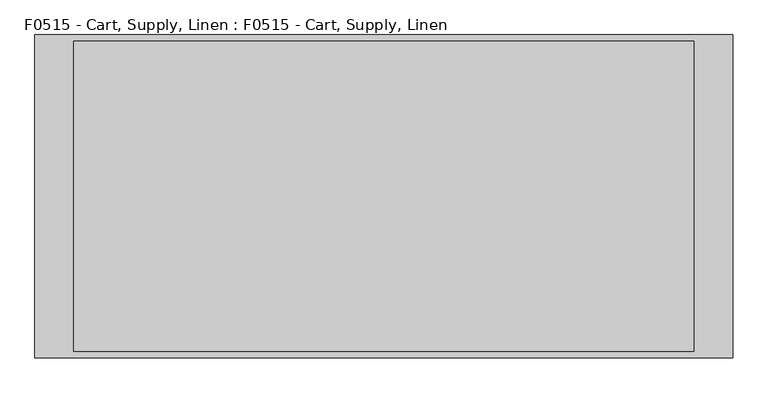
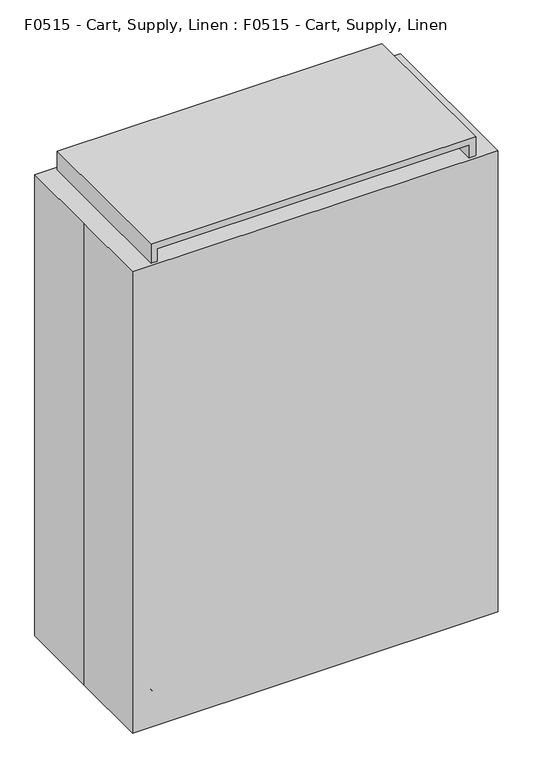
"""IFC4 building model written with IfcOpenShell, lengths in millimetres: proxy geometry, F0515 - Cart, Supply, Linen : F0515 - Cart, Supply, Linen."""

import ifcopenshell
import ifcopenshell.guid

model = None  # the IFC model being written
_history = None  # IfcOwnerHistory: only IFC2X3 demands one
_inside = {}  # id of a spatial element -> (the spatial element, [elements in it])
_under = {}  # id of a project, library or spatial element -> (it, [spatial elements below it])
_declared = {}  # id of a project -> (the project, [libraries it declares])
_typed = {}  # id of a type object -> (the type object, [elements of that type])
_made_of = {}  # id of a material, layer set ... -> (it, [elements and type objects made of it])


def new_model(schema):
    """Start an empty IFC model of exactly this schema.

    Asked for "IFC4X3", IfcOpenShell would pick the latest addendum, in which some entities
    have other attributes; the version numbers below select the first issue.
    IFC2X3 requires an IfcOwnerHistory on every rooted entity: one is made here for all.
    """
    global model, _history
    if schema == "IFC4X3":
        model = ifcopenshell.file(schema_version=(4, 3, 0, 0))
    else:
        model = ifcopenshell.file(schema=schema)
    _inside.clear()
    _under.clear()
    _declared.clear()
    _typed.clear()
    _made_of.clear()
    _history = None
    if model.schema == "IFC2X3":
        org = make("IfcOrganization", Name="unknown")
        user = make(
            "IfcPersonAndOrganization",
            ThePerson=make("IfcPerson", FamilyName="unknown"),
            TheOrganization=org,
        )
        app = make(
            "IfcApplication",
            ApplicationDeveloper=org,
            Version="unknown",
            ApplicationFullName="unknown",
            ApplicationIdentifier="unknown",
        )
        _history = make(
            "IfcOwnerHistory",
            OwningUser=user,
            OwningApplication=app,
            ChangeAction="ADDED",
            CreationDate=0,
        )
    return model


def make(cls, **values):
    """One entity of the class cls with the attributes given. An attribute that is None is left unset."""
    return model.create_entity(
        cls, **{name: value for name, value in values.items() if value is not None}
    )


def rooted(cls, **values):
    """An entity with a GlobalId (a new one), such as an element, a storey or a relation."""
    return make(cls, GlobalId=ifcopenshell.guid.new(), OwnerHistory=_history, **values)


def si_unit(unit_type, name, prefix=None):
    """IfcSIUnit, for example si_unit("LENGTHUNIT", "METRE", prefix="MILLI")."""
    return make("IfcSIUnit", UnitType=unit_type, Prefix=prefix, Name=name)


def assignment(units):
    """IfcUnitAssignment: the units of a project."""
    return None if units is None else make("IfcUnitAssignment", Units=units)


def point(xyz):
    """IfcCartesianPoint."""
    return None if xyz is None else make("IfcCartesianPoint", Coordinates=xyz)


def direction(xyz):
    """IfcDirection."""
    return None if xyz is None else make("IfcDirection", DirectionRatios=xyz)


def frame(location, z_axis=None, x_axis=None):
    """IfcAxis2Placement3D, a coordinate frame: its origin and axes. An axis left out is left unset."""
    return make(
        "IfcAxis2Placement3D",
        Location=point(location),
        Axis=direction(z_axis),
        RefDirection=direction(x_axis),
    )


def frame_2d(location, x_axis=None):
    """IfcAxis2Placement2D, a coordinate frame in the plane: its origin and x axis."""
    return make(
        "IfcAxis2Placement2D", Location=point(location), RefDirection=direction(x_axis)
    )


def origin():
    """The frame at (0, 0, 0) with its axes left unset."""
    return frame((0.0, 0.0, 0.0))


def origin_with_axes():
    """The frame at (0, 0, 0) with the z axis (0, 0, 1) and the x axis (1, 0, 0) written out."""
    return frame((0.0, 0.0, 0.0), z_axis=(0.0, 0.0, 1.0), x_axis=(1.0, 0.0, 0.0))


def place(relative_to, where):
    """IfcLocalPlacement: puts the frame where relative to a parent placement (None: the world)."""
    return make(
        "IfcLocalPlacement", PlacementRelTo=relative_to, RelativePlacement=where
    )


def context(
    kind, dimensions, precision=None, world=None, true_north=None, identifier=None
):
    """IfcGeometricRepresentationContext, for example the 3D "Model" context."""
    return make(
        "IfcGeometricRepresentationContext",
        ContextIdentifier=identifier,
        ContextType=kind,
        CoordinateSpaceDimension=dimensions,
        Precision=precision,
        WorldCoordinateSystem=world,
        TrueNorth=true_north,
    )


def project(units=None, contexts=None):
    """IfcProject with its units and contexts."""
    return rooted(
        "IfcProject",
        Name="project",
        RepresentationContexts=contexts,
        UnitsInContext=assignment(units),
    )


def spatial(cls, under=None, at=None, **own):
    """A site, building, storey or space (cls), placed at a placement, below another one or the project."""
    s = rooted(cls, ObjectPlacement=at, **own)
    if under is not None:
        _under.setdefault(under.id(), (under, []))[1].append(s)
    return s


def polyline(points):
    """IfcPolyline through the points."""
    return make("IfcPolyline", Points=[point(p) for p in points])


def circle_curve(where, radius):
    """IfcCircle in the frame where."""
    return make("IfcCircle", Position=where, Radius=radius)


def trimmed(basis, trim1, trim2, sense, master):
    """IfcTrimmedCurve: the piece of a basis curve between two trims."""
    return make(
        "IfcTrimmedCurve",
        BasisCurve=basis,
        Trim1=trim1,
        Trim2=trim2,
        SenseAgreement=sense,
        MasterRepresentation=master,
    )


def segment(curve, same_sense, transition):
    """IfcCompositeCurveSegment."""
    return make(
        "IfcCompositeCurveSegment",
        Transition=transition,
        SameSense=same_sense,
        ParentCurve=curve,
    )


def composite_curve(segments, self_intersect=None):
    """IfcCompositeCurve: segments joined end to end."""
    return make("IfcCompositeCurve", Segments=segments, SelfIntersect=self_intersect)


def outline(outer, holes=None, kind="AREA"):
    """IfcArbitraryClosedProfileDef: a profile drawn as a closed curve; with holes, ...WithVoids."""
    if holes is None:
        return make("IfcArbitraryClosedProfileDef", ProfileType=kind, OuterCurve=outer)
    return make(
        "IfcArbitraryProfileDefWithVoids",
        ProfileType=kind,
        OuterCurve=outer,
        InnerCurves=holes,
    )


def extrude(swept, where, along, depth):
    """IfcExtrudedAreaSolid: the profile swept, set in the frame where, extruded along a direction by depth."""
    return make(
        "IfcExtrudedAreaSolid",
        SweptArea=swept,
        Position=where,
        ExtrudedDirection=direction(along),
        Depth=depth,
    )


def faces_of(points, faces, orient=None, outer=None):
    """IfcFace entities. A face is a list of loops; a loop is a list of indices into points, from 0.

    orient and outer hold one flag for each loop. By default every Orientation is true, the
    first loop of a face is its IfcFaceOuterBound and the others are IfcFaceBound.
    """
    made = []
    for i, loops in enumerate(faces):
        bounds = []
        for j, loop in enumerate(loops):
            is_outer = j == 0 if outer is None else outer[i][j]
            bounds.append(
                make(
                    "IfcFaceOuterBound" if is_outer else "IfcFaceBound",
                    Bound=make("IfcPolyLoop", Polygon=[points[k] for k in loop]),
                    Orientation=True if orient is None else orient[i][j],
                )
            )
        made.append(make("IfcFace", Bounds=bounds))
    return made


def faceted_brep(points, faces, orient=None, outer=None, voids=None):
    """IfcFacetedBrep: a solid bounded by flat faces; with voids (closed shells), ...WithVoids."""
    shared = [point(p) for p in points]
    hull = make("IfcClosedShell", CfsFaces=faces_of(shared, faces, orient, outer))
    if voids is None:
        return make("IfcFacetedBrep", Outer=hull)
    return make(
        "IfcFacetedBrepWithVoids",
        Outer=hull,
        Voids=[
            make(cls, CfsFaces=faces_of(shared, fs, o, b)) for cls, fs, o, b in voids
        ],
    )


def shape(context_of_items, identifier, shape_type, items):
    """IfcShapeRepresentation: the items that make up one representation, for example the "Body"."""
    return make(
        "IfcShapeRepresentation",
        ContextOfItems=context_of_items,
        RepresentationIdentifier=identifier,
        RepresentationType=shape_type,
        Items=items,
    )


def source(mapping_origin, context_of_items, identifier, shape_type, items):
    """IfcRepresentationMap: a shape defined once, which mapped items show again and again."""
    return make(
        "IfcRepresentationMap",
        MappingOrigin=mapping_origin,
        MappedRepresentation=shape(context_of_items, identifier, shape_type, items),
    )


def transform(
    local_origin,
    x_axis=None,
    y_axis=None,
    z_axis=None,
    scale=None,
    scale2=None,
    scale3=None,
    uniform=True,
):
    """IfcCartesianTransformationOperator3D, or its non-uniform kind. x_axis, y_axis, z_axis: its Axis1, 2, 3."""
    if uniform:
        return make(
            "IfcCartesianTransformationOperator3D",
            Axis1=direction(x_axis),
            Axis2=direction(y_axis),
            LocalOrigin=point(local_origin),
            Scale=scale,
            Axis3=direction(z_axis),
        )
    return make(
        "IfcCartesianTransformationOperator3DnonUniform",
        Axis1=direction(x_axis),
        Axis2=direction(y_axis),
        LocalOrigin=point(local_origin),
        Scale=scale,
        Axis3=direction(z_axis),
        Scale2=scale2,
        Scale3=scale3,
    )


def mapped(mapping_source, mapping_target):
    """IfcMappedItem: shows the shape of a source again, moved by a transform."""
    return make(
        "IfcMappedItem", MappingSource=mapping_source, MappingTarget=mapping_target
    )


def made_of(thing, what):
    """Note that an element or type object is made of a material, layer set ...; save() writes the relation."""
    if what is not None:
        _made_of.setdefault(what.id(), (what, []))[1].append(thing)
    return thing


def element(
    cls,
    number,
    at=None,
    inside=None,
    cuts=None,
    type_object=None,
    material=None,
    context=None,
    identifier="Body",
    shape_type=None,
    held_by="IfcProductDefinitionShape",
    body=None,
    shapes=None,
    **own,
):
    """One element of the class cls, such as IfcWall. Its Tag is "e" and its number.

    at: its placement. inside: the storey or other place that contains it. cuts: it is an
    opening in that element (IfcRelVoidsElement). A single representation is given by context,
    identifier, shape_type and body (its items); several are given by shapes. held_by: the class
    of the entity that holds the representations. save() writes the other relations.
    """
    e = rooted(cls, Tag="e%d" % number, ObjectPlacement=at, **own)
    if body is not None:
        shapes = [shape(context, identifier, shape_type, body)]
    if shapes is not None:
        e.Representation = make(held_by, Representations=shapes)
    if inside is not None:
        _inside.setdefault(inside.id(), (inside, []))[1].append(e)
    if cuts is not None:
        rooted(
            "IfcRelVoidsElement", RelatingBuildingElement=cuts, RelatedOpeningElement=e
        )
    if type_object is not None:
        _typed.setdefault(type_object.id(), (type_object, []))[1].append(e)
    return made_of(e, material)


def aggregate(whole, parts):
    """IfcRelAggregates: a whole, such as a stair, and the parts it consists of."""
    return rooted("IfcRelAggregates", RelatingObject=whole, RelatedObjects=parts)


def save(model, path):
    """Write the relations noted so far, then the file.

    IfcRelAggregates (storeys below a building ...), IfcRelContainedInSpatialStructure (elements
    in a storey), IfcRelDefinesByType, IfcRelAssociatesMaterial and IfcRelDeclares: one each for
    every whole, place, type object, material and project.
    """
    for whole, parts in _under.values():
        aggregate(whole, parts)
    for where, things in _inside.values():
        rooted(
            "IfcRelContainedInSpatialStructure",
            RelatedElements=things,
            RelatingStructure=where,
        )
    for kind, things in _typed.values():
        rooted("IfcRelDefinesByType", RelatedObjects=things, RelatingType=kind)
    for what, things in _made_of.values():
        rooted("IfcRelAssociatesMaterial", RelatedObjects=things, RelatingMaterial=what)
    for by, libraries in _declared.values():
        rooted("IfcRelDeclares", RelatingContext=by, RelatedDefinitions=libraries)
    model.write(path)


def f0515_cart_supply_linen_f0515_cart_supply_linen_772906bd(model_context):
    return source(origin(), model_context, "Body", "SolidModel", [
        extrude(outline(polyline([(138.1125, 609.6), (138.1125, 496.8875), (60.3746094, 542.8753906), (60.3746094, 555.5753906), (138.1125, 609.6)])), frame((0.0, 241.3, 0.0), z_axis=(0.0, 1.0, 0.0), x_axis=(0.0, 0.0, 1.0)), (0.0, 0.0, 1.0), 3.175),
        extrude(outline(polyline([(138.1125, 609.6), (138.1125, 496.8875), (60.3746094, 542.8753906), (60.3746094, 555.5753906), (138.1125, 609.6)])), frame((0.0, 263.525, 0.0), z_axis=(0.0, 1.0, 0.0), x_axis=(0.0, 0.0, 1.0)), (0.0, 0.0, 1.0), 3.175),
        extrude(outline(composite_curve([segment(trimmed(circle_curve(frame_2d((60.3746094, 549.2253906)), 60.3746094), [point((60.3746094, 609.6))], [point((60.3746094, 488.8507812))], False, "CARTESIAN"), True, "CONTINUOUS"), segment(trimmed(circle_curve(frame_2d((60.3746094, 549.2253906)), 60.3746094), [point((60.3746094, 488.8507812))], [point((60.3746094, 609.6))], False, "CARTESIAN"), True, "CONTINUOUS")], self_intersect=False)), frame((0.0, 244.475, 0.0), z_axis=(0.0, 1.0, 0.0), x_axis=(0.0, 0.0, 1.0)), (0.0, 0.0, 1.0), 19.05),
        extrude(outline(composite_curve([segment(trimmed(circle_curve(frame_2d((584.2, 279.4)), 25.4), [point((584.2, 304.8))], [point((609.6, 279.4))], False, "CARTESIAN"), True, "CONTINUOUS"), segment(polyline([(609.6, 279.4), (609.6, 228.6)]), True, "CONTINUOUS"), segment(trimmed(circle_curve(frame_2d((584.2, 228.6)), 25.4), [point((609.6, 228.6))], [point((584.2, 203.2))], False, "CARTESIAN"), True, "CONTINUOUS"), segment(polyline([(584.2, 203.2), (533.4, 203.2)]), True, "CONTINUOUS"), segment(trimmed(circle_curve(frame_2d((533.4, 228.6)), 25.4), [point((533.4, 203.2))], [point((508.0, 228.6))], False, "CARTESIAN"), True, "CONTINUOUS"), segment(polyline([(508.0, 228.6), (508.0, 279.4)]), True, "CONTINUOUS"), segment(trimmed(circle_curve(frame_2d((533.4, 279.4)), 25.4), [point((508.0, 279.4))], [point((533.4, 304.8))], False, "CARTESIAN"), True, "CONTINUOUS"), segment(polyline([(533.4, 304.8), (584.2, 304.8)]), True, "CONTINUOUS")], self_intersect=False)), frame((0.0, 0.0, 138.1125), z_axis=(0.0, 0.0, 1.0), x_axis=(1.0, 0.0, 0.0)), (0.0, 0.0, 1.0), 25.4),
        extrude(outline(polyline([(138.1125, -609.6), (60.3746094, -555.5753906), (60.3746094, -542.8753906), (138.1125, -496.8875), (138.1125, -609.6)])), frame((0.0, 241.3, 0.0), z_axis=(0.0, 1.0, 0.0), x_axis=(0.0, 0.0, 1.0)), (0.0, 0.0, 1.0), 3.175),
        extrude(outline(polyline([(138.1125, -609.6), (60.3746094, -555.5753906), (60.3746094, -542.8753906), (138.1125, -496.8875), (138.1125, -609.6)])), frame((0.0, 263.525, 0.0), z_axis=(0.0, 1.0, 0.0), x_axis=(0.0, 0.0, 1.0)), (0.0, 0.0, 1.0), 3.175),
        extrude(outline(composite_curve([segment(trimmed(circle_curve(frame_2d((60.3746094, -549.2253906)), 60.3746094), [point((60.3746094, -609.6))], [point((60.3746094, -488.8507812))], False, "CARTESIAN"), True, "CONTINUOUS"), segment(trimmed(circle_curve(frame_2d((60.3746094, -549.2253906)), 60.3746094), [point((60.3746094, -488.8507812))], [point((60.3746094, -609.6))], False, "CARTESIAN"), True, "CONTINUOUS")], self_intersect=False)), frame((0.0, 244.475, 0.0), z_axis=(0.0, 1.0, 0.0), x_axis=(0.0, 0.0, 1.0)), (0.0, 0.0, 1.0), 19.05),
        extrude(outline(composite_curve([segment(polyline([(-584.2, 304.8), (-533.4, 304.8)]), True, "CONTINUOUS"), segment(trimmed(circle_curve(frame_2d((-533.4, 279.4)), 25.4), [point((-533.4, 304.8))], [point((-508.0, 279.4))], False, "CARTESIAN"), True, "CONTINUOUS"), segment(polyline([(-508.0, 279.4), (-508.0, 228.6)]), True, "CONTINUOUS"), segment(trimmed(circle_curve(frame_2d((-533.4, 228.6)), 25.4), [point((-508.0, 228.6))], [point((-533.4, 203.2))], False, "CARTESIAN"), True, "CONTINUOUS"), segment(polyline([(-533.4, 203.2), (-584.2, 203.2)]), True, "CONTINUOUS"), segment(trimmed(circle_curve(frame_2d((-584.2, 228.6)), 25.4), [point((-584.2, 203.2))], [point((-609.6, 228.6))], False, "CARTESIAN"), True, "CONTINUOUS"), segment(polyline([(-609.6, 228.6), (-609.6, 279.4)]), True, "CONTINUOUS"), segment(trimmed(circle_curve(frame_2d((-584.2, 279.4)), 25.4), [point((-609.6, 279.4))], [point((-584.2, 304.8))], False, "CARTESIAN"), True, "CONTINUOUS")], self_intersect=False)), frame((0.0, 0.0, 138.1125), z_axis=(0.0, 0.0, 1.0), x_axis=(1.0, 0.0, 0.0)), (0.0, 0.0, 1.0), 25.4),
        extrude(outline(polyline([(138.1125, 609.6), (138.1125, 496.8875), (60.3746094, 542.8753906), (60.3746094, 555.5753906), (138.1125, 609.6)])), frame((0.0, -244.475, 0.0), z_axis=(0.0, 1.0, 0.0), x_axis=(0.0, 0.0, 1.0)), (0.0, 0.0, 1.0), 3.175),
        extrude(outline(polyline([(138.1125, 609.6), (138.1125, 496.8875), (60.3746094, 542.8753906), (60.3746094, 555.5753906), (138.1125, 609.6)])), frame((0.0, -266.7, 0.0), z_axis=(0.0, 1.0, 0.0), x_axis=(0.0, 0.0, 1.0)), (0.0, 0.0, 1.0), 3.175),
        extrude(outline(composite_curve([segment(trimmed(circle_curve(frame_2d((60.3746094, 549.2253906)), 60.3746094), [point((60.3746094, 609.6))], [point((60.3746094, 488.8507812))], False, "CARTESIAN"), True, "CONTINUOUS"), segment(trimmed(circle_curve(frame_2d((60.3746094, 549.2253906)), 60.3746094), [point((60.3746094, 488.8507812))], [point((60.3746094, 609.6))], False, "CARTESIAN"), True, "CONTINUOUS")], self_intersect=False)), frame((0.0, -263.525, 0.0), z_axis=(0.0, 1.0, 0.0), x_axis=(0.0, 0.0, 1.0)), (0.0, 0.0, 1.0), 19.05),
        extrude(outline(composite_curve([segment(polyline([(584.2, -304.8), (533.4, -304.8)]), True, "CONTINUOUS"), segment(trimmed(circle_curve(frame_2d((533.4, -279.4)), 25.4), [point((533.4, -304.8))], [point((508.0, -279.4))], False, "CARTESIAN"), True, "CONTINUOUS"), segment(polyline([(508.0, -279.4), (508.0, -228.6)]), True, "CONTINUOUS"), segment(trimmed(circle_curve(frame_2d((533.4, -228.6)), 25.4), [point((508.0, -228.6))], [point((533.4, -203.2))], False, "CARTESIAN"), True, "CONTINUOUS"), segment(polyline([(533.4, -203.2), (584.2, -203.2)]), True, "CONTINUOUS"), segment(trimmed(circle_curve(frame_2d((584.2, -228.6)), 25.4), [point((584.2, -203.2))], [point((609.6, -228.6))], False, "CARTESIAN"), True, "CONTINUOUS"), segment(polyline([(609.6, -228.6), (609.6, -279.4)]), True, "CONTINUOUS"), segment(trimmed(circle_curve(frame_2d((584.2, -279.4)), 25.4), [point((609.6, -279.4))], [point((584.2, -304.8))], False, "CARTESIAN"), True, "CONTINUOUS")], self_intersect=False)), frame((0.0, 0.0, 138.1125), z_axis=(0.0, 0.0, 1.0), x_axis=(1.0, 0.0, 0.0)), (0.0, 0.0, 1.0), 25.4),
        extrude(outline(polyline([(138.1125, -609.6), (60.3746094, -555.5753906), (60.3746094, -542.8753906), (138.1125, -496.8875), (138.1125, -609.6)])), frame((0.0, -244.475, 0.0), z_axis=(0.0, 1.0, 0.0), x_axis=(0.0, 0.0, 1.0)), (0.0, 0.0, 1.0), 3.175),
        extrude(outline(polyline([(138.1125, -609.6), (60.3746094, -555.5753906), (60.3746094, -542.8753906), (138.1125, -496.8875), (138.1125, -609.6)])), frame((0.0, -266.7, 0.0), z_axis=(0.0, 1.0, 0.0), x_axis=(0.0, 0.0, 1.0)), (0.0, 0.0, 1.0), 3.175),
        extrude(outline(composite_curve([segment(trimmed(circle_curve(frame_2d((60.3746094, -549.2253906)), 60.3746094), [point((60.3746094, -609.6))], [point((60.3746094, -488.8507812))], False, "CARTESIAN"), True, "CONTINUOUS"), segment(trimmed(circle_curve(frame_2d((60.3746094, -549.2253906)), 60.3746094), [point((60.3746094, -488.8507812))], [point((60.3746094, -609.6))], False, "CARTESIAN"), True, "CONTINUOUS")], self_intersect=False)), frame((0.0, -263.525, 0.0), z_axis=(0.0, 1.0, 0.0), x_axis=(0.0, 0.0, 1.0)), (0.0, 0.0, 1.0), 19.05),
        extrude(outline(composite_curve([segment(trimmed(circle_curve(frame_2d((-584.2, -279.4)), 25.4), [point((-584.2, -304.8))], [point((-609.6, -279.4))], False, "CARTESIAN"), True, "CONTINUOUS"), segment(polyline([(-609.6, -279.4), (-609.6, -228.6)]), True, "CONTINUOUS"), segment(trimmed(circle_curve(frame_2d((-584.2, -228.6)), 25.4), [point((-609.6, -228.6))], [point((-584.2, -203.2))], False, "CARTESIAN"), True, "CONTINUOUS"), segment(polyline([(-584.2, -203.2), (-533.4, -203.2)]), True, "CONTINUOUS"), segment(trimmed(circle_curve(frame_2d((-533.4, -228.6)), 25.4), [point((-533.4, -203.2))], [point((-508.0, -228.6))], False, "CARTESIAN"), True, "CONTINUOUS"), segment(polyline([(-508.0, -228.6), (-508.0, -279.4)]), True, "CONTINUOUS"), segment(trimmed(circle_curve(frame_2d((-533.4, -279.4)), 25.4), [point((-508.0, -279.4))], [point((-533.4, -304.8))], False, "CARTESIAN"), True, "CONTINUOUS"), segment(polyline([(-533.4, -304.8), (-584.2, -304.8)]), True, "CONTINUOUS")], self_intersect=False)), frame((0.0, 0.0, 138.1125), z_axis=(0.0, 0.0, 1.0), x_axis=(1.0, 0.0, 0.0)), (0.0, 0.0, 1.0), 25.4),
        faceted_brep([(-609.6, -304.8, 163.5125), (609.6, -304.8, 163.5125), (609.6, -304.8, 1903.4125), (-609.6, -304.8, 1903.4125), (584.2, -304.8, 1878.0125), (584.2, -304.8, 1568.1325), (-584.2, -304.8, 1568.1325), (-584.2, -304.8, 1878.0125), (-584.2, -304.8, 498.7925), (584.2, -304.8, 498.7925), (584.2, -304.8, 188.9125), (-584.2, -304.8, 188.9125), (584.2, -304.8, 1542.7325), (584.2, -304.8, 1220.1525), (-584.2, -304.8, 1220.1525), (-584.2, -304.8, 1542.7325), (584.2, -304.8, 1194.7525), (584.2, -304.8, 872.1725), (-584.2, -304.8, 872.1725), (-584.2, -304.8, 1194.7525), (584.2, -304.8, 846.7725), (584.2, -304.8, 524.1925), (-584.2, -304.8, 524.1925), (-584.2, -304.8, 846.7725), (-609.6, 304.8, 163.5125), (609.6, 304.8, 163.5125), (609.6, 304.8, 1903.4125), (-609.6, 304.8, 1903.4125), (584.2, 279.4, 1878.0125), (584.2, 279.4, 1568.1325), (-584.2, 279.4, 1568.1325), (-584.2, 279.4, 1878.0125), (-584.2, 279.4, 498.7925), (584.2, 279.4, 498.7925), (584.2, 279.4, 188.9125), (-584.2, 279.4, 188.9125), (584.2, 279.4, 1542.7325), (584.2, 279.4, 1220.1525), (-584.2, 279.4, 1220.1525), (-584.2, 279.4, 1542.7325), (584.2, 279.4, 1194.7525), (584.2, 279.4, 872.1725), (-584.2, 279.4, 872.1725), (-584.2, 279.4, 1194.7525), (584.2, 279.4, 846.7725), (584.2, 279.4, 524.1925), (-584.2, 279.4, 524.1925), (-584.2, 279.4, 846.7725)], [[[0, 1, 2, 3], [4, 5, 6, 7], [8, 9, 10, 11], [12, 13, 14, 15], [16, 17, 18, 19], [20, 21, 22, 23]], [[1, 0, 24, 25]], [[2, 1, 25, 26]], [[3, 2, 26, 27]], [[24, 0, 3, 27]], [[5, 4, 28, 29]], [[6, 5, 29, 30]], [[7, 6, 30, 31]], [[4, 7, 31, 28]], [[9, 8, 32, 33]], [[10, 9, 33, 34]], [[11, 10, 34, 35]], [[8, 11, 35, 32]], [[13, 12, 36, 37]], [[14, 13, 37, 38]], [[15, 14, 38, 39]], [[12, 15, 39, 36]], [[17, 16, 40, 41]], [[18, 17, 41, 42]], [[19, 18, 42, 43]], [[16, 19, 43, 40]], [[21, 20, 44, 45]], [[22, 21, 45, 46]], [[23, 22, 46, 47]], [[20, 23, 47, 44]], [[27, 26, 25, 24]], [[29, 28, 31, 30]], [[33, 32, 35, 34]], [[37, 36, 39, 38]], [[41, 40, 43, 42]], [[45, 44, 47, 46]]]),
        extrude(outline(polyline([(-685.8, 317.5), (685.8, 317.5), (685.8, -317.5), (-685.8, -317.5), (-685.8, 0.0), (-685.8, 317.5)])), origin_with_axes(), (0.0, 0.0, 1.0), 1828.8),
    ])


if __name__ == "__main__":
    model = new_model("IFC4")
    model_context = context("Model", 3, world=origin())
    ifc_project = project(units=[si_unit("LENGTHUNIT", "METRE", prefix="MILLI")], contexts=[model_context])
    site = spatial("IfcSite", under=ifc_project)
    building = spatial("IfcBuilding", under=site)
    placement = place(None, origin())
    f0515_cart_supply_linen_f0515_cart_supply_linen_shape = f0515_cart_supply_linen_f0515_cart_supply_linen_772906bd(model_context)
    element("IfcBuildingElementProxy", 1, Name="F0515 - Cart, Supply, Linen : F0515 - Cart, Supply, Linen", ObjectType="F0515 - Cart, Supply, Linen : F0515 - Cart, Supply, Linen", at=placement, inside=building, context=model_context, shape_type="MappedRepresentation", body=[
        mapped(f0515_cart_supply_linen_f0515_cart_supply_linen_shape, transform((0.0, 0.0, 0.0), x_axis=(1.0, 0.0, 0.0), y_axis=(0.0, 1.0, 0.0), z_axis=(0.0, 0.0, 1.0))),
    ])
    save(model, "model.ifc")

# Revit data of these elements
# Project information
#   Room Abbreviation = "NBCD5"
#   Room Description = "Decontamination Patient Transition (NBCD5)"
#   Sheets - Total = "6"
#   Project Issue Date = "Issue Date"
#   Project Status = "Project Status"
#   Client Name = "Owner"
#   Project Address = "Enter address here"
#   Project Name = "Project Name"
#   Project Number = "Project Number"
#   Publication Date = "30-Jan-15"
# Type "F0515 - Cart, Supply, Linen : F0515 - Cart, Supply, Linen"
#   Watts2 = "0"
#   Watts1 = "0"
#   Unit_Issue = "EA"
#   UTIL_6_Misc = "-"
#   UTIL_5_NonMedGas = "-"
#   UTIL_4_MiscGas = "-"
#   UTIL_3_MedGas = "-"
#   UTIL_2_Elec = "-"
#   UTIL_1_WaterDrain = "-"
#   Nomenclature = "Cart, Supply, Linen"
#   NSN = "7100"
#   Location [instance default] = ""
#   JSN = "F0515"
#   Fund_Source_VA = "-"
#   Fund_Source_Navy = "-"
#   Fund_Source_Army = "-"
#   Fund_Source_AF = "-"
#   ELEC_Volts2 = "0"
#   ELEC_Volts1 = "0"
#   ELEC_Phase2 = "0"
#   ELEC_Phase1 = "0"
#   ELEC_HertzSwitch = "0"
#   ELEC_HertzDependent = "0"
#   ELEC_Hertz = "0"
#   ELEC_Amps2 = "0"
#   ELEC_Amps1 = "0"
#   DetailDescription = "Closed linen supply cart. Equipped with four (4) non-marking rubber tire roller bearing casters and heavy duty cover. May be used for the delivery and user storage of clean linen as well as the return of soiled linen."
#   CAT_VA = "C"
#   CAT_Navy = "C"
#   CAT_IHS = "-"
#   CAT_Army = "C"
#   CAT_AF = "C"
#   BTUperhour = "0"
#   Weight_IP = 205
#   DIM_Width_IP = 4' - 6"
#   DIM_Height_IP = 6' - 0"
#   DIM_Depth_IP = 2' - 1"
# Element 1 (IfcBuildingElementProxy, "F0515 - Cart, Supply, Linen : F0515 - Cart, Supply, Linen")
#   Materials on its faces: "Herman Miller - Finish LU Soft White", "Wheel Material", "EquipSpace"
# Materials
#   "Herman Miller - Finish LU Soft White": class "Plastic", colour RGB 245 239 218, transparency 0
#   "Wheel Material": class "Plastic", colour RGB 5 5 5, transparency 0
#   "EquipSpace": class "Unassigned", colour RGB 221 217 195, transparency 0.5
